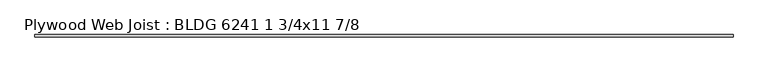
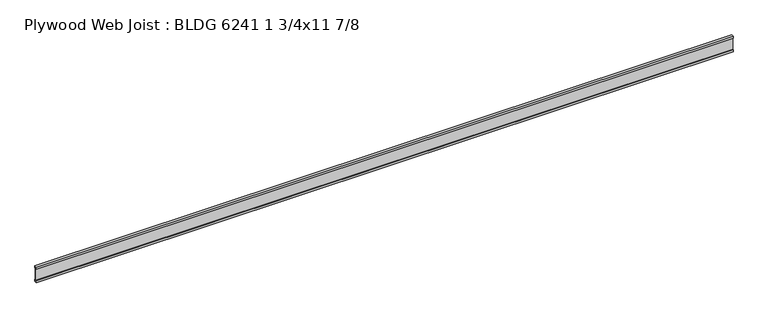
"""IFC4 building model written with IfcOpenShell, lengths in millimetres: beam geometry, Plywood Web Joist : BLDG 6241 1 3/4x11 7/8."""

import ifcopenshell
import ifcopenshell.guid

model = None  # the IFC model being written
_history = None  # IfcOwnerHistory: only IFC2X3 demands one
_inside = {}  # id of a spatial element -> (the spatial element, [elements in it])
_under = {}  # id of a project, library or spatial element -> (it, [spatial elements below it])
_declared = {}  # id of a project -> (the project, [libraries it declares])
_typed = {}  # id of a type object -> (the type object, [elements of that type])
_made_of = {}  # id of a material, layer set ... -> (it, [elements and type objects made of it])


def new_model(schema):
    """Start an empty IFC model of exactly this schema.

    Asked for "IFC4X3", IfcOpenShell would pick the latest addendum, in which some entities
    have other attributes; the version numbers below select the first issue.
    IFC2X3 requires an IfcOwnerHistory on every rooted entity: one is made here for all.
    """
    global model, _history
    if schema == "IFC4X3":
        model = ifcopenshell.file(schema_version=(4, 3, 0, 0))
    else:
        model = ifcopenshell.file(schema=schema)
    _inside.clear()
    _under.clear()
    _declared.clear()
    _typed.clear()
    _made_of.clear()
    _history = None
    if model.schema == "IFC2X3":
        org = make("IfcOrganization", Name="unknown")
        user = make(
            "IfcPersonAndOrganization",
            ThePerson=make("IfcPerson", FamilyName="unknown"),
            TheOrganization=org,
        )
        app = make(
            "IfcApplication",
            ApplicationDeveloper=org,
            Version="unknown",
            ApplicationFullName="unknown",
            ApplicationIdentifier="unknown",
        )
        _history = make(
            "IfcOwnerHistory",
            OwningUser=user,
            OwningApplication=app,
            ChangeAction="ADDED",
            CreationDate=0,
        )
    return model


def make(cls, **values):
    """One entity of the class cls with the attributes given. An attribute that is None is left unset."""
    return model.create_entity(
        cls, **{name: value for name, value in values.items() if value is not None}
    )


def rooted(cls, **values):
    """An entity with a GlobalId (a new one), such as an element, a storey or a relation."""
    return make(cls, GlobalId=ifcopenshell.guid.new(), OwnerHistory=_history, **values)


def si_unit(unit_type, name, prefix=None):
    """IfcSIUnit, for example si_unit("LENGTHUNIT", "METRE", prefix="MILLI")."""
    return make("IfcSIUnit", UnitType=unit_type, Prefix=prefix, Name=name)


def assignment(units):
    """IfcUnitAssignment: the units of a project."""
    return None if units is None else make("IfcUnitAssignment", Units=units)


def point(xyz):
    """IfcCartesianPoint."""
    return None if xyz is None else make("IfcCartesianPoint", Coordinates=xyz)


def direction(xyz):
    """IfcDirection."""
    return None if xyz is None else make("IfcDirection", DirectionRatios=xyz)


def frame(location, z_axis=None, x_axis=None):
    """IfcAxis2Placement3D, a coordinate frame: its origin and axes. An axis left out is left unset."""
    return make(
        "IfcAxis2Placement3D",
        Location=point(location),
        Axis=direction(z_axis),
        RefDirection=direction(x_axis),
    )


def origin():
    """The frame at (0, 0, 0) with its axes left unset."""
    return frame((0.0, 0.0, 0.0))


def place(relative_to, where):
    """IfcLocalPlacement: puts the frame where relative to a parent placement (None: the world)."""
    return make(
        "IfcLocalPlacement", PlacementRelTo=relative_to, RelativePlacement=where
    )


def context(
    kind, dimensions, precision=None, world=None, true_north=None, identifier=None
):
    """IfcGeometricRepresentationContext, for example the 3D "Model" context."""
    return make(
        "IfcGeometricRepresentationContext",
        ContextIdentifier=identifier,
        ContextType=kind,
        CoordinateSpaceDimension=dimensions,
        Precision=precision,
        WorldCoordinateSystem=world,
        TrueNorth=true_north,
    )


def project(units=None, contexts=None):
    """IfcProject with its units and contexts."""
    return rooted(
        "IfcProject",
        Name="project",
        RepresentationContexts=contexts,
        UnitsInContext=assignment(units),
    )


def spatial(cls, under=None, at=None, **own):
    """A site, building, storey or space (cls), placed at a placement, below another one or the project."""
    s = rooted(cls, ObjectPlacement=at, **own)
    if under is not None:
        _under.setdefault(under.id(), (under, []))[1].append(s)
    return s


def polyline(points):
    """IfcPolyline through the points."""
    return make("IfcPolyline", Points=[point(p) for p in points])


def outline(outer, holes=None, kind="AREA"):
    """IfcArbitraryClosedProfileDef: a profile drawn as a closed curve; with holes, ...WithVoids."""
    if holes is None:
        return make("IfcArbitraryClosedProfileDef", ProfileType=kind, OuterCurve=outer)
    return make(
        "IfcArbitraryProfileDefWithVoids",
        ProfileType=kind,
        OuterCurve=outer,
        InnerCurves=holes,
    )


def extrude(swept, where, along, depth):
    """IfcExtrudedAreaSolid: the profile swept, set in the frame where, extruded along a direction by depth."""
    return make(
        "IfcExtrudedAreaSolid",
        SweptArea=swept,
        Position=where,
        ExtrudedDirection=direction(along),
        Depth=depth,
    )


def shape(context_of_items, identifier, shape_type, items):
    """IfcShapeRepresentation: the items that make up one representation, for example the "Body"."""
    return make(
        "IfcShapeRepresentation",
        ContextOfItems=context_of_items,
        RepresentationIdentifier=identifier,
        RepresentationType=shape_type,
        Items=items,
    )


def source(mapping_origin, context_of_items, identifier, shape_type, items):
    """IfcRepresentationMap: a shape defined once, which mapped items show again and again."""
    return make(
        "IfcRepresentationMap",
        MappingOrigin=mapping_origin,
        MappedRepresentation=shape(context_of_items, identifier, shape_type, items),
    )


def transform(
    local_origin,
    x_axis=None,
    y_axis=None,
    z_axis=None,
    scale=None,
    scale2=None,
    scale3=None,
    uniform=True,
):
    """IfcCartesianTransformationOperator3D, or its non-uniform kind. x_axis, y_axis, z_axis: its Axis1, 2, 3."""
    if uniform:
        return make(
            "IfcCartesianTransformationOperator3D",
            Axis1=direction(x_axis),
            Axis2=direction(y_axis),
            LocalOrigin=point(local_origin),
            Scale=scale,
            Axis3=direction(z_axis),
        )
    return make(
        "IfcCartesianTransformationOperator3DnonUniform",
        Axis1=direction(x_axis),
        Axis2=direction(y_axis),
        LocalOrigin=point(local_origin),
        Scale=scale,
        Axis3=direction(z_axis),
        Scale2=scale2,
        Scale3=scale3,
    )


def mapped(mapping_source, mapping_target):
    """IfcMappedItem: shows the shape of a source again, moved by a transform."""
    return make(
        "IfcMappedItem", MappingSource=mapping_source, MappingTarget=mapping_target
    )


def made_of(thing, what):
    """Note that an element or type object is made of a material, layer set ...; save() writes the relation."""
    if what is not None:
        _made_of.setdefault(what.id(), (what, []))[1].append(thing)
    return thing


def element(
    cls,
    number,
    at=None,
    inside=None,
    cuts=None,
    type_object=None,
    material=None,
    context=None,
    identifier="Body",
    shape_type=None,
    held_by="IfcProductDefinitionShape",
    body=None,
    shapes=None,
    **own,
):
    """One element of the class cls, such as IfcWall. Its Tag is "e" and its number.

    at: its placement. inside: the storey or other place that contains it. cuts: it is an
    opening in that element (IfcRelVoidsElement). A single representation is given by context,
    identifier, shape_type and body (its items); several are given by shapes. held_by: the class
    of the entity that holds the representations. save() writes the other relations.
    """
    e = rooted(cls, Tag="e%d" % number, ObjectPlacement=at, **own)
    if body is not None:
        shapes = [shape(context, identifier, shape_type, body)]
    if shapes is not None:
        e.Representation = make(held_by, Representations=shapes)
    if inside is not None:
        _inside.setdefault(inside.id(), (inside, []))[1].append(e)
    if cuts is not None:
        rooted(
            "IfcRelVoidsElement", RelatingBuildingElement=cuts, RelatedOpeningElement=e
        )
    if type_object is not None:
        _typed.setdefault(type_object.id(), (type_object, []))[1].append(e)
    return made_of(e, material)


def aggregate(whole, parts):
    """IfcRelAggregates: a whole, such as a stair, and the parts it consists of."""
    return rooted("IfcRelAggregates", RelatingObject=whole, RelatedObjects=parts)


def save(model, path):
    """Write the relations noted so far, then the file.

    IfcRelAggregates (storeys below a building ...), IfcRelContainedInSpatialStructure (elements
    in a storey), IfcRelDefinesByType, IfcRelAssociatesMaterial and IfcRelDeclares: one each for
    every whole, place, type object, material and project.
    """
    for whole, parts in _under.values():
        aggregate(whole, parts)
    for where, things in _inside.values():
        rooted(
            "IfcRelContainedInSpatialStructure",
            RelatedElements=things,
            RelatingStructure=where,
        )
    for kind, things in _typed.values():
        rooted("IfcRelDefinesByType", RelatedObjects=things, RelatingType=kind)
    for what, things in _made_of.values():
        rooted("IfcRelAssociatesMaterial", RelatedObjects=things, RelatingMaterial=what)
    for by, libraries in _declared.values():
        rooted("IfcRelDeclares", RelatingContext=by, RelatedDefinitions=libraries)
    model.write(path)


def plywood_web_joist_bldg_6241_1_3_4x11_7_8_0dbcbf17(model_context):
    return source(origin(), model_context, "Body", "SweptSolid", [
        extrude(outline(polyline([(-22.225, 150.8125), (22.225, 150.8125), (22.225, 112.7125), (4.7625, 112.7125), (4.7625, 119.0625), (-4.7625, 119.0625), (-4.7625, 112.7125), (-22.225, 112.7125), (-22.225, 150.8125)])), frame((-6365.875, 0.0, 0.0), z_axis=(1.0, 0.0, 0.0), x_axis=(0.0, 1.0, 0.0)), (0.0, 0.0, 1.0), 12731.75),
        extrude(outline(polyline([(22.225, -112.7125), (22.225, -150.8125), (-22.225, -150.8125), (-22.225, -112.7125), (-4.7625, -112.7125), (-4.7625, -118.3285374), (4.7625, -118.3285374), (4.7625, -112.7125), (22.225, -112.7125)])), frame((-6365.875, 0.0, 0.0), z_axis=(1.0, 0.0, 0.0), x_axis=(0.0, 1.0, 0.0)), (0.0, 0.0, 1.0), 12731.75),
        extrude(outline(polyline([(6365.875, 4.7625), (6365.875, -4.7625), (-6365.875, -4.7625), (-6365.875, 4.7625), (6365.875, 4.7625)])), frame((0.0, 0.0, -118.3285374), z_axis=(0.0, 0.0, 1.0), x_axis=(1.0, 0.0, 0.0)), (0.0, 0.0, 1.0), 237.3910374),
    ])


if __name__ == "__main__":
    model = new_model("IFC4")
    model_context = context("Model", 3, world=origin())
    ifc_project = project(units=[si_unit("LENGTHUNIT", "METRE", prefix="MILLI")], contexts=[model_context])
    site = spatial("IfcSite", under=ifc_project)
    building = spatial("IfcBuilding", under=site)
    placement = place(None, origin())
    plywood_web_joist_bldg_6241_1_3_4x11_7_8_shape = plywood_web_joist_bldg_6241_1_3_4x11_7_8_0dbcbf17(model_context)
    element("IfcBeam", 1, ObjectType="Plywood Web Joist : BLDG 6241 1 3/4x11 7/8", at=placement, inside=building, context=model_context, shape_type="MappedRepresentation", body=[
        mapped(plywood_web_joist_bldg_6241_1_3_4x11_7_8_shape, transform((0.0, 0.0, 0.0), x_axis=(1.0, 0.0, 0.0), y_axis=(0.0, 1.0, 0.0), z_axis=(0.0, 0.0, 1.0))),
    ])
    save(model, "model.ifc")

# Revit data of these elements
# Type "Plywood Web Joist : BLDG 6241 1 3/4x11 7/8"
#   Assembly Code = "B10"
#   Length [instance default] = 5' - 0"
#   b = 0' - 1 3/4"
#   d = 0' - 11 7/8"
#   Structural Material [instance default] = Softwood, Lumber
# Element 1 (IfcBeam, "Plywood Web Joist : BLDG 6241 1 3/4x11 7/8")
#   Materials on its faces: "Softwood, Lumber"
# Materials
#   "Softwood, Lumber": class "Wood", colour RGB 223 192 134, transparency 0, Description = "Pinus Echinata", Cost = 0
